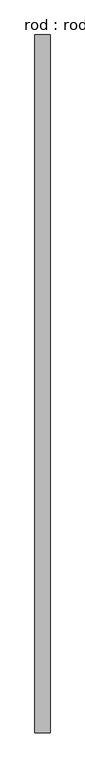
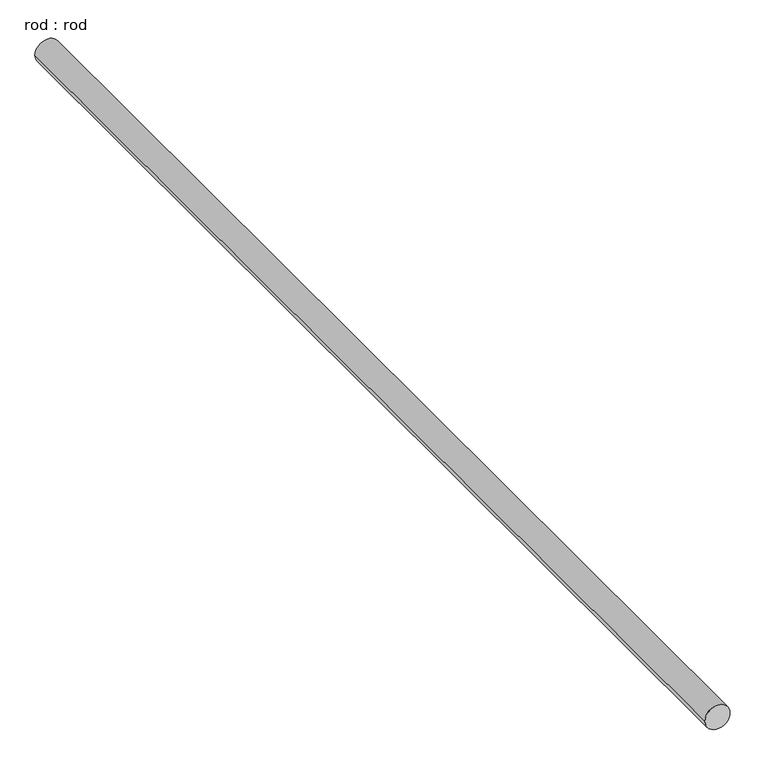
"""IFC4 building model written with IfcOpenShell, lengths in millimetres: proxy geometry, rod : rod."""

from ifc_helpers import new_model, si_unit, point, frame, frame_2d, origin, place, context, project, spatial, circle_curve, trimmed, segment, composite_curve, outline, extrude, source, transform, mapped, element, save


def rod_rod_76b85bc7(model_context):
    return source(origin(), model_context, "Body", "SweptSolid", [
        extrude(outline(composite_curve([segment(trimmed(circle_curve(frame_2d((0.0108462, 0.0)), 200.0), [point((0.0108462, 200.0))], [point((0.0108462, -200.0))], False, "CARTESIAN"), True, "CONTINUOUS"), segment(trimmed(circle_curve(frame_2d((0.0108462, 0.0)), 200.0), [point((0.0108462, -200.0))], [point((0.0108462, 200.0))], False, "CARTESIAN"), True, "CONTINUOUS")], self_intersect=False)), frame((0.0, -5129.7577963, 0.0), z_axis=(0.0, 1.0, 0.0), x_axis=(0.0, 0.0, 1.0)), (0.0, 0.0, 1.0), 18444.9728232),
    ])


if __name__ == "__main__":
    model = new_model("IFC4")
    model_context = context("Model", 3, world=origin())
    ifc_project = project(units=[si_unit("LENGTHUNIT", "METRE", prefix="MILLI")], contexts=[model_context])
    site = spatial("IfcSite", under=ifc_project)
    building = spatial("IfcBuilding", under=site)
    placement = place(None, origin())
    rod_rod_shape = rod_rod_76b85bc7(model_context)
    element("IfcBuildingElementProxy", 1, Name="rod : rod", ObjectType="rod : rod", at=placement, inside=building, context=model_context, shape_type="MappedRepresentation", body=[
        mapped(rod_rod_shape, transform((0.0, 0.0, 0.0), x_axis=(1.0, 0.0, 0.0), y_axis=(0.0, 1.0, 0.0), z_axis=(0.0, 0.0, 1.0))),
    ])
    save(model, "model.ifc")

# Revit data of these elements
# Type "rod : rod"
#   Default Elevation = 0
